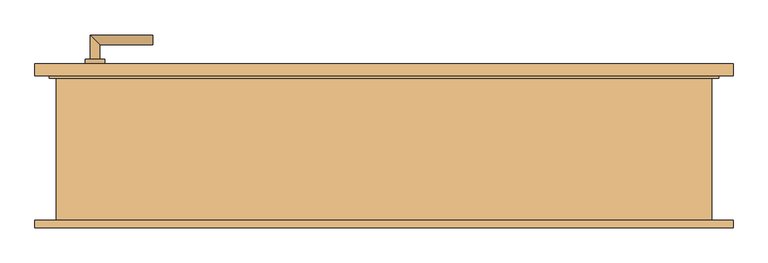
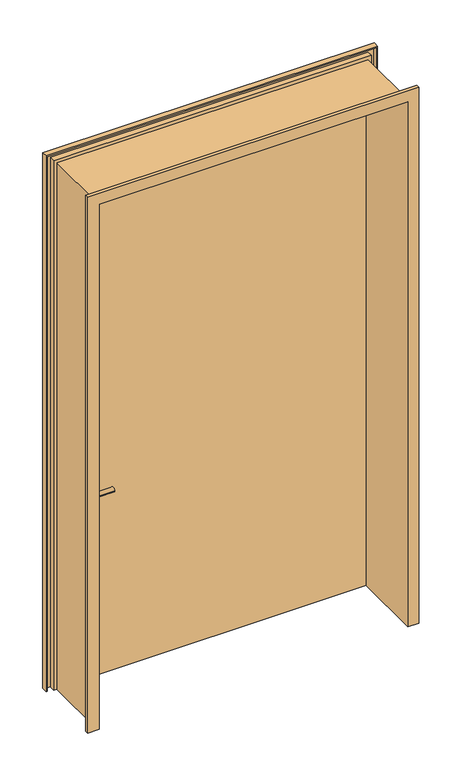
"""IFC4 building model written with IfcOpenShell, lengths in millimetres: door geometry, Drehflügel 1-flg - Stahlzarge : Holztüre 1,4 x 2,45 2."""

import ifcopenshell
import ifcopenshell.guid

model = None  # the IFC model being written
_history = None  # IfcOwnerHistory: only IFC2X3 demands one
_inside = {}  # id of a spatial element -> (the spatial element, [elements in it])
_under = {}  # id of a project, library or spatial element -> (it, [spatial elements below it])
_declared = {}  # id of a project -> (the project, [libraries it declares])
_typed = {}  # id of a type object -> (the type object, [elements of that type])
_made_of = {}  # id of a material, layer set ... -> (it, [elements and type objects made of it])


def new_model(schema):
    """Start an empty IFC model of exactly this schema.

    Asked for "IFC4X3", IfcOpenShell would pick the latest addendum, in which some entities
    have other attributes; the version numbers below select the first issue.
    IFC2X3 requires an IfcOwnerHistory on every rooted entity: one is made here for all.
    """
    global model, _history
    if schema == "IFC4X3":
        model = ifcopenshell.file(schema_version=(4, 3, 0, 0))
    else:
        model = ifcopenshell.file(schema=schema)
    _inside.clear()
    _under.clear()
    _declared.clear()
    _typed.clear()
    _made_of.clear()
    _history = None
    if model.schema == "IFC2X3":
        org = make("IfcOrganization", Name="unknown")
        user = make(
            "IfcPersonAndOrganization",
            ThePerson=make("IfcPerson", FamilyName="unknown"),
            TheOrganization=org,
        )
        app = make(
            "IfcApplication",
            ApplicationDeveloper=org,
            Version="unknown",
            ApplicationFullName="unknown",
            ApplicationIdentifier="unknown",
        )
        _history = make(
            "IfcOwnerHistory",
            OwningUser=user,
            OwningApplication=app,
            ChangeAction="ADDED",
            CreationDate=0,
        )
    return model


def make(cls, **values):
    """One entity of the class cls with the attributes given. An attribute that is None is left unset."""
    return model.create_entity(
        cls, **{name: value for name, value in values.items() if value is not None}
    )


def rooted(cls, **values):
    """An entity with a GlobalId (a new one), such as an element, a storey or a relation."""
    return make(cls, GlobalId=ifcopenshell.guid.new(), OwnerHistory=_history, **values)


def si_unit(unit_type, name, prefix=None):
    """IfcSIUnit, for example si_unit("LENGTHUNIT", "METRE", prefix="MILLI")."""
    return make("IfcSIUnit", UnitType=unit_type, Prefix=prefix, Name=name)


def assignment(units):
    """IfcUnitAssignment: the units of a project."""
    return None if units is None else make("IfcUnitAssignment", Units=units)


def point(xyz):
    """IfcCartesianPoint."""
    return None if xyz is None else make("IfcCartesianPoint", Coordinates=xyz)


def direction(xyz):
    """IfcDirection."""
    return None if xyz is None else make("IfcDirection", DirectionRatios=xyz)


def frame(location, z_axis=None, x_axis=None):
    """IfcAxis2Placement3D, a coordinate frame: its origin and axes. An axis left out is left unset."""
    return make(
        "IfcAxis2Placement3D",
        Location=point(location),
        Axis=direction(z_axis),
        RefDirection=direction(x_axis),
    )


def frame_2d(location, x_axis=None):
    """IfcAxis2Placement2D, a coordinate frame in the plane: its origin and x axis."""
    return make(
        "IfcAxis2Placement2D", Location=point(location), RefDirection=direction(x_axis)
    )


def origin():
    """The frame at (0, 0, 0) with its axes left unset."""
    return frame((0.0, 0.0, 0.0))


def place(relative_to, where):
    """IfcLocalPlacement: puts the frame where relative to a parent placement (None: the world)."""
    return make(
        "IfcLocalPlacement", PlacementRelTo=relative_to, RelativePlacement=where
    )


def context(
    kind, dimensions, precision=None, world=None, true_north=None, identifier=None
):
    """IfcGeometricRepresentationContext, for example the 3D "Model" context."""
    return make(
        "IfcGeometricRepresentationContext",
        ContextIdentifier=identifier,
        ContextType=kind,
        CoordinateSpaceDimension=dimensions,
        Precision=precision,
        WorldCoordinateSystem=world,
        TrueNorth=true_north,
    )


def project(units=None, contexts=None):
    """IfcProject with its units and contexts."""
    return rooted(
        "IfcProject",
        Name="project",
        RepresentationContexts=contexts,
        UnitsInContext=assignment(units),
    )


def spatial(cls, under=None, at=None, **own):
    """A site, building, storey or space (cls), placed at a placement, below another one or the project."""
    s = rooted(cls, ObjectPlacement=at, **own)
    if under is not None:
        _under.setdefault(under.id(), (under, []))[1].append(s)
    return s


def polyline(points):
    """IfcPolyline through the points."""
    return make("IfcPolyline", Points=[point(p) for p in points])


def circle_curve(where, radius):
    """IfcCircle in the frame where."""
    return make("IfcCircle", Position=where, Radius=radius)


def ellipse_curve(where, semi_axis1, semi_axis2):
    """IfcEllipse in the frame where."""
    return make(
        "IfcEllipse", Position=where, SemiAxis1=semi_axis1, SemiAxis2=semi_axis2
    )


def trimmed(basis, trim1, trim2, sense, master):
    """IfcTrimmedCurve: the piece of a basis curve between two trims."""
    return make(
        "IfcTrimmedCurve",
        BasisCurve=basis,
        Trim1=trim1,
        Trim2=trim2,
        SenseAgreement=sense,
        MasterRepresentation=master,
    )


def segment(curve, same_sense, transition):
    """IfcCompositeCurveSegment."""
    return make(
        "IfcCompositeCurveSegment",
        Transition=transition,
        SameSense=same_sense,
        ParentCurve=curve,
    )


def composite_curve(segments, self_intersect=None):
    """IfcCompositeCurve: segments joined end to end."""
    return make("IfcCompositeCurve", Segments=segments, SelfIntersect=self_intersect)


def outline(outer, holes=None, kind="AREA"):
    """IfcArbitraryClosedProfileDef: a profile drawn as a closed curve; with holes, ...WithVoids."""
    if holes is None:
        return make("IfcArbitraryClosedProfileDef", ProfileType=kind, OuterCurve=outer)
    return make(
        "IfcArbitraryProfileDefWithVoids",
        ProfileType=kind,
        OuterCurve=outer,
        InnerCurves=holes,
    )


def extrude(swept, where, along, depth):
    """IfcExtrudedAreaSolid: the profile swept, set in the frame where, extruded along a direction by depth."""
    return make(
        "IfcExtrudedAreaSolid",
        SweptArea=swept,
        Position=where,
        ExtrudedDirection=direction(along),
        Depth=depth,
    )


def faces_of(points, faces, orient=None, outer=None):
    """IfcFace entities. A face is a list of loops; a loop is a list of indices into points, from 0.

    orient and outer hold one flag for each loop. By default every Orientation is true, the
    first loop of a face is its IfcFaceOuterBound and the others are IfcFaceBound.
    """
    made = []
    for i, loops in enumerate(faces):
        bounds = []
        for j, loop in enumerate(loops):
            is_outer = j == 0 if outer is None else outer[i][j]
            bounds.append(
                make(
                    "IfcFaceOuterBound" if is_outer else "IfcFaceBound",
                    Bound=make("IfcPolyLoop", Polygon=[points[k] for k in loop]),
                    Orientation=True if orient is None else orient[i][j],
                )
            )
        made.append(make("IfcFace", Bounds=bounds))
    return made


def faceted_brep(points, faces, orient=None, outer=None, voids=None):
    """IfcFacetedBrep: a solid bounded by flat faces; with voids (closed shells), ...WithVoids."""
    shared = [point(p) for p in points]
    hull = make("IfcClosedShell", CfsFaces=faces_of(shared, faces, orient, outer))
    if voids is None:
        return make("IfcFacetedBrep", Outer=hull)
    return make(
        "IfcFacetedBrepWithVoids",
        Outer=hull,
        Voids=[
            make(cls, CfsFaces=faces_of(shared, fs, o, b)) for cls, fs, o, b in voids
        ],
    )


def shape(context_of_items, identifier, shape_type, items):
    """IfcShapeRepresentation: the items that make up one representation, for example the "Body"."""
    return make(
        "IfcShapeRepresentation",
        ContextOfItems=context_of_items,
        RepresentationIdentifier=identifier,
        RepresentationType=shape_type,
        Items=items,
    )


def source(mapping_origin, context_of_items, identifier, shape_type, items):
    """IfcRepresentationMap: a shape defined once, which mapped items show again and again."""
    return make(
        "IfcRepresentationMap",
        MappingOrigin=mapping_origin,
        MappedRepresentation=shape(context_of_items, identifier, shape_type, items),
    )


def transform(
    local_origin,
    x_axis=None,
    y_axis=None,
    z_axis=None,
    scale=None,
    scale2=None,
    scale3=None,
    uniform=True,
):
    """IfcCartesianTransformationOperator3D, or its non-uniform kind. x_axis, y_axis, z_axis: its Axis1, 2, 3."""
    if uniform:
        return make(
            "IfcCartesianTransformationOperator3D",
            Axis1=direction(x_axis),
            Axis2=direction(y_axis),
            LocalOrigin=point(local_origin),
            Scale=scale,
            Axis3=direction(z_axis),
        )
    return make(
        "IfcCartesianTransformationOperator3DnonUniform",
        Axis1=direction(x_axis),
        Axis2=direction(y_axis),
        LocalOrigin=point(local_origin),
        Scale=scale,
        Axis3=direction(z_axis),
        Scale2=scale2,
        Scale3=scale3,
    )


def mapped(mapping_source, mapping_target):
    """IfcMappedItem: shows the shape of a source again, moved by a transform."""
    return make(
        "IfcMappedItem", MappingSource=mapping_source, MappingTarget=mapping_target
    )


def made_of(thing, what):
    """Note that an element or type object is made of a material, layer set ...; save() writes the relation."""
    if what is not None:
        _made_of.setdefault(what.id(), (what, []))[1].append(thing)
    return thing


def element(
    cls,
    number,
    at=None,
    inside=None,
    cuts=None,
    type_object=None,
    material=None,
    context=None,
    identifier="Body",
    shape_type=None,
    held_by="IfcProductDefinitionShape",
    body=None,
    shapes=None,
    **own,
):
    """One element of the class cls, such as IfcWall. Its Tag is "e" and its number.

    at: its placement. inside: the storey or other place that contains it. cuts: it is an
    opening in that element (IfcRelVoidsElement). A single representation is given by context,
    identifier, shape_type and body (its items); several are given by shapes. held_by: the class
    of the entity that holds the representations. save() writes the other relations.
    """
    e = rooted(cls, Tag="e%d" % number, ObjectPlacement=at, **own)
    if body is not None:
        shapes = [shape(context, identifier, shape_type, body)]
    if shapes is not None:
        e.Representation = make(held_by, Representations=shapes)
    if inside is not None:
        _inside.setdefault(inside.id(), (inside, []))[1].append(e)
    if cuts is not None:
        rooted(
            "IfcRelVoidsElement", RelatingBuildingElement=cuts, RelatedOpeningElement=e
        )
    if type_object is not None:
        _typed.setdefault(type_object.id(), (type_object, []))[1].append(e)
    return made_of(e, material)


def aggregate(whole, parts):
    """IfcRelAggregates: a whole, such as a stair, and the parts it consists of."""
    return rooted("IfcRelAggregates", RelatingObject=whole, RelatedObjects=parts)


def save(model, path):
    """Write the relations noted so far, then the file.

    IfcRelAggregates (storeys below a building ...), IfcRelContainedInSpatialStructure (elements
    in a storey), IfcRelDefinesByType, IfcRelAssociatesMaterial and IfcRelDeclares: one each for
    every whole, place, type object, material and project.
    """
    for whole, parts in _under.values():
        aggregate(whole, parts)
    for where, things in _inside.values():
        rooted(
            "IfcRelContainedInSpatialStructure",
            RelatedElements=things,
            RelatingStructure=where,
        )
    for kind, things in _typed.values():
        rooted("IfcRelDefinesByType", RelatedObjects=things, RelatingType=kind)
    for what, things in _made_of.values():
        rooted("IfcRelAssociatesMaterial", RelatedObjects=things, RelatingMaterial=what)
    for by, libraries in _declared.values():
        rooted("IfcRelDeclares", RelatingContext=by, RelatedDefinitions=libraries)
    model.write(path)


def plane_surface(at):
    """IfcPlane: the flat surface through the origin of the frame at, square to its z axis."""
    return make("IfcPlane", Position=at)


def cylinder_surface(at, radius):
    """IfcCylindricalSurface: all points at the distance radius from the z axis of the frame at."""
    return make("IfcCylindricalSurface", Position=at, Radius=radius)


def advanced_brep(points, edges, surfaces, faces):
    """IfcAdvancedBrep: a solid bounded by faces that lie on surfaces and meet in shared edges.

    An edge is (start, end): straight between two places in points (the first is 0);
    or (start, end, curve); or (start, end, curve, False) where it runs against its curve.
    A face is (place in surfaces, loops), or (place, loops, False) where it looks against
    its surface's normal. A loop lists edges by number (the first is 1), with a minus sign
    where the edge is run from its end to its start. The first loop is the outer one.
    """
    corners = [point(p) for p in points]
    vertices = [make("IfcVertexPoint", VertexGeometry=c) for c in corners]
    made = []
    for start, end, *more in edges:
        made.append(
            make(
                "IfcEdgeCurve",
                EdgeStart=vertices[start],
                EdgeEnd=vertices[end],
                EdgeGeometry=more[0] if more else make("IfcPolyline", Points=[corners[start], corners[end]]),
                SameSense=more[1] if len(more) > 1 else True,
            )
        )
    hull = []
    for where, loops, *sense in faces:
        bounds = []
        for j, loop in enumerate(loops):
            ring = [make("IfcOrientedEdge", EdgeElement=made[abs(k) - 1], Orientation=k > 0) for k in loop]
            bounds.append(
                make(
                    "IfcFaceOuterBound" if j == 0 else "IfcFaceBound",
                    Bound=make("IfcEdgeLoop", EdgeList=ring),
                    Orientation=True,
                )
            )
        hull.append(make("IfcAdvancedFace", Bounds=bounds, FaceSurface=surfaces[where], SameSense=sense[0] if sense else True))
    return make("IfcAdvancedBrep", Outer=make("IfcClosedShell", CfsFaces=hull))


def door_901329f2(model_context):
    return source(origin(), model_context, "Body", "SolidModel", [
        advanced_brep(
        [(-610.0, 139.4346141, 1000.0), (-590.0, 139.4346141, 1000.0), (-610.0, 69.4346141, 1000.0), (-590.0, 89.4346141, 1000.0), (-480.0, 69.4346141, 1000.0), (-480.0, 89.4346141, 1000.0)],
        [
            (0, 1, circle_curve(frame((-600.0, 139.4346141, 1000.0), z_axis=(0.0, 1.0, 0.0), x_axis=(1.0, 0.0, 0.0)), 10.0)),
            (1, 0, circle_curve(frame((-600.0, 139.4346141, 1000.0), z_axis=(0.0, 1.0, 0.0), x_axis=(1.0, 0.0, 0.0)), 10.0)),
            (0, 2),
            (2, 3, ellipse_curve(frame((-600.0, 79.4346141, 1000.0), z_axis=(-0.7071067811865385, 0.7071067811865565, 0.0), x_axis=(0.7071067811865563, 0.7071067811865386, 0.0)), 14.1421356, 10.0)),
            (3, 1),
            (3, 2, ellipse_curve(frame((-600.0, 79.4346141, 1000.0), z_axis=(-0.7071067811865385, 0.7071067811865565, 0.0), x_axis=(0.7071067811865563, 0.7071067811865386, 0.0)), 14.1421356, 10.0)),
            (4, 5, circle_curve(frame((-480.0, 79.4346141, 1000.0), z_axis=(1.0, 0.0, 0.0), x_axis=(0.0, 1.0, 0.0)), 10.0)),
            (5, 4, circle_curve(frame((-480.0, 79.4346141, 1000.0), z_axis=(1.0, 0.0, 0.0), x_axis=(0.0, 1.0, 0.0)), 10.0)),
            (2, 4),
            (5, 3),
        ],
        [
            plane_surface(frame((-600.0, 139.4346141, -287.7526403), z_axis=(0.0, 1.0, 0.0), x_axis=(0.0, 0.0, 1.0))),
            cylinder_surface(frame((-600.0, 139.4346141, 1000.0), z_axis=(0.0, 1.0, 0.0), x_axis=(1.0, 0.0, 0.0)), 10.0),
            plane_surface(frame((-480.0, 79.4346141, -287.7526403), z_axis=(1.0, 0.0, 0.0), x_axis=(0.0, 0.0, 1.0))),
            cylinder_surface(frame((-600.0, 79.4346141, 1000.0), z_axis=(-1.0, 0.0, 0.0), x_axis=(0.0, 1.0, 0.0)), 10.0),
        ],
        [
            (0, [[1, 2]]),
            (1, [[-1, 3, 4, 5]]),
            (1, [[-2, -5, 6, -3]]),
            (2, [[7, 8]]),
            (3, [[-4, 9, -8, 10]]),
            (3, [[-6, -10, -7, -9]]),
        ],
    ),
        advanced_brep(
        [(-590.0, 199.4346141, 1000.0), (-610.0, 199.4346141, 1000.0), (-590.0, 229.4346141, 1000.0), (-610.0, 249.4346141, 1000.0), (-480.0, 229.4346141, 1000.0), (-480.0, 249.4346141, 1000.0)],
        [
            (0, 1, circle_curve(frame((-600.0, 199.4346141, 1000.0), z_axis=(0.0, -1.0, 0.0), x_axis=(-1.0, 0.0, 0.0)), 10.0)),
            (1, 0, circle_curve(frame((-600.0, 199.4346141, 1000.0), z_axis=(0.0, -1.0, 0.0), x_axis=(-1.0, 0.0, 0.0)), 10.0)),
            (0, 2),
            (2, 3, ellipse_curve(frame((-600.0, 239.4346141, 1000.0), z_axis=(-0.7071067811865475, -0.7071067811865475, 0.0), x_axis=(0.7071067811865474, -0.7071067811865476, 0.0)), 14.1421356, 10.0)),
            (3, 1),
            (3, 2, ellipse_curve(frame((-600.0, 239.4346141, 1000.0), z_axis=(-0.7071067811865475, -0.7071067811865475, 0.0), x_axis=(0.7071067811865474, -0.7071067811865476, 0.0)), 14.1421356, 10.0)),
            (4, 5, circle_curve(frame((-480.0, 239.4346141, 1000.0), z_axis=(1.0, 0.0, 0.0), x_axis=(0.0, 1.0, 0.0)), 10.0)),
            (5, 4, circle_curve(frame((-480.0, 239.4346141, 1000.0), z_axis=(1.0, 0.0, 0.0), x_axis=(0.0, 1.0, 0.0)), 10.0)),
            (2, 4),
            (5, 3),
        ],
        [
            plane_surface(frame((-600.0, 199.4346141, -287.7526403), z_axis=(0.0, -1.0, 0.0), x_axis=(0.0, 0.0, 1.0))),
            cylinder_surface(frame((-600.0, 199.4346141, 1000.0), z_axis=(0.0, -1.0, 0.0), x_axis=(-1.0, 0.0, 0.0)), 10.0),
            plane_surface(frame((-480.0, 239.4346141, -287.7526403), z_axis=(1.0, 0.0, 0.0), x_axis=(0.0, 0.0, 1.0))),
            cylinder_surface(frame((-600.0, 239.4346141, 1000.0), z_axis=(-1.0, 0.0, 0.0), x_axis=(0.0, 1.0, 0.0)), 10.0),
        ],
        [
            (0, [[1, 2]]),
            (1, [[-1, 3, 4, 5]]),
            (1, [[-2, -5, 6, -3]]),
            (2, [[7, 8]]),
            (3, [[-4, 9, -8, 10]]),
            (3, [[-6, -10, -7, -9]]),
        ],
    ),
        extrude(outline(composite_curve([segment(trimmed(circle_curve(frame_2d((1000.0, -600.0)), 20.0), [point((1000.0, -620.0))], [point((1000.0, -580.0))], False, "CARTESIAN"), True, "CONTINUOUS"), segment(trimmed(circle_curve(frame_2d((1000.0, -600.0)), 20.0), [point((1000.0, -580.0))], [point((1000.0, -620.0))], False, "CARTESIAN"), True, "CONTINUOUS")], self_intersect=False)), frame((0.0, 129.4346141, 0.0), z_axis=(0.0, 1.0, 0.0), x_axis=(0.0, 0.0, 1.0)), (0.0, 0.0, 1.0), 10.0),
        extrude(outline(composite_curve([segment(trimmed(circle_curve(frame_2d((1000.0, -600.0)), 20.0), [point((1000.0, -620.0))], [point((1000.0, -580.0))], False, "CARTESIAN"), True, "CONTINUOUS"), segment(trimmed(circle_curve(frame_2d((1000.0, -600.0)), 20.0), [point((1000.0, -580.0))], [point((1000.0, -620.0))], False, "CARTESIAN"), True, "CONTINUOUS")], self_intersect=False)), frame((0.0, 189.4346141, 0.0), z_axis=(0.0, 1.0, 0.0), x_axis=(0.0, 0.0, 1.0)), (0.0, 0.0, 1.0), 10.0),
        extrude(outline(polyline([(690.0, 164.4346141), (-690.0, 164.4346141), (-690.0, 189.4346141), (690.0, 189.4346141), (690.0, 164.4346141)])), frame((0.0, 0.0, 100.0), z_axis=(0.0, 0.0, 1.0), x_axis=(1.0, 0.0, 0.0)), (0.0, 0.0, 1.0), 2440.0),
        faceted_brep([(724.4603207, -150.5653859, 100.0), (675.0, -150.5653859, 100.0), (675.0, 164.4346141, 100.0), (690.0, 164.4346141, 100.0), (690.0, 189.4346141, 100.0), (724.4603207, 189.4346141, 100.0), (724.4603207, 164.4346141, 100.0), (719.4603207, 164.4346141, 100.0), (719.4603207, 184.4346141, 100.0), (695.0, 184.4346141, 100.0), (695.0, 159.4346141, 100.0), (680.0, 159.4346141, 100.0), (680.0, -145.5653859, 100.0), (719.4603207, -145.5653859, 100.0), (719.4603207, -135.5653859, 100.0), (724.4603207, -135.5653859, 100.0), (724.4603207, -150.5653859, 2574.4603207), (-724.4603207, -150.5653859, 2574.4603207), (-724.4603207, -150.5653859, 100.0), (-675.0, -150.5653859, 100.0), (-675.0, -150.5653859, 2525.0), (675.0, -150.5653859, 2525.0), (675.0, 164.4346141, 2525.0), (-675.0, 164.4346141, 2525.0), (-675.0, 164.4346141, 100.0), (-690.0, 164.4346141, 100.0), (-690.0, 164.4346141, 2540.0), (690.0, 164.4346141, 2540.0), (690.0, 189.4346141, 2540.0), (-690.0, 189.4346141, 2540.0), (-690.0, 189.4346141, 100.0), (-724.4603207, 189.4346141, 100.0), (-724.4603207, 189.4346141, 2574.4603207), (724.4603207, 189.4346141, 2574.4603207), (724.4603207, 164.4346141, 2574.4603207), (-724.4603207, 164.4346141, 2574.4603207), (-724.4603207, 164.4346141, 100.0), (-719.4603207, 164.4346141, 100.0), (-719.4603207, 164.4346141, 2569.4603207), (719.4603207, 164.4346141, 2569.4603207), (719.4603207, 184.4346141, 2569.4603207), (-719.4603207, 184.4346141, 2569.4603207), (-719.4603207, 184.4346141, 100.0), (-695.0, 184.4346141, 100.0), (-695.0, 184.4346141, 2545.0), (695.0, 184.4346141, 2545.0), (695.0, 159.4346141, 2545.0), (-695.0, 159.4346141, 2545.0), (-695.0, 159.4346141, 100.0), (-680.0, 159.4346141, 100.0), (-680.0, 159.4346141, 2530.0), (680.0, 159.4346141, 2530.0), (680.0, -145.5653859, 2530.0), (-680.0, -145.5653859, 2530.0), (-680.0, -145.5653859, 100.0), (-719.4603207, -145.5653859, 100.0), (-719.4603207, -145.5653859, 2569.4603207), (719.4603207, -145.5653859, 2569.4603207), (719.4603207, -135.5653859, 2569.4603207), (-719.4603207, -135.5653859, 2569.4603207), (-719.4603207, -135.5653859, 100.0), (-724.4603207, -135.5653859, 100.0), (-724.4603207, -135.5653859, 2574.4603207), (724.4603207, -135.5653859, 2574.4603207)], [[[0, 1, 2, 3, 4, 5, 6, 7, 8, 9, 10, 11, 12, 13, 14, 15]], [[1, 0, 16, 17, 18, 19, 20, 21]], [[2, 1, 21, 22]], [[3, 2, 22, 23, 24, 25, 26, 27]], [[4, 3, 27, 28]], [[5, 4, 28, 29, 30, 31, 32, 33]], [[6, 5, 33, 34]], [[7, 6, 34, 35, 36, 37, 38, 39]], [[8, 7, 39, 40]], [[9, 8, 40, 41, 42, 43, 44, 45]], [[10, 9, 45, 46]], [[11, 10, 46, 47, 48, 49, 50, 51]], [[12, 11, 51, 52]], [[13, 12, 52, 53, 54, 55, 56, 57]], [[14, 13, 57, 58]], [[15, 14, 58, 59, 60, 61, 62, 63]], [[0, 15, 63, 16]], [[17, 62, 61, 18]], [[18, 61, 60, 55, 54, 49, 48, 43, 42, 37, 36, 31, 30, 25, 24, 19]], [[23, 20, 19, 24]], [[29, 26, 25, 30]], [[35, 32, 31, 36]], [[41, 38, 37, 42]], [[47, 44, 43, 48]], [[53, 50, 49, 54]], [[59, 56, 55, 60]], [[22, 21, 20, 23]], [[28, 27, 26, 29]], [[34, 33, 32, 35]], [[40, 39, 38, 41]], [[46, 45, 44, 47]], [[52, 51, 50, 53]], [[58, 57, 56, 59]], [[16, 63, 62, 17]]]),
    ])


if __name__ == "__main__":
    model = new_model("IFC4")
    model_context = context("Model", 3, world=origin())
    ifc_project = project(units=[si_unit("LENGTHUNIT", "METRE", prefix="MILLI")], contexts=[model_context])
    site = spatial("IfcSite", under=ifc_project)
    building = spatial("IfcBuilding", under=site)
    placement = place(None, origin())
    door_shape = door_901329f2(model_context)
    element("IfcDoor", 1, ObjectType="Drehflügel 1-flg - Stahlzarge : Holztüre 1,4 x 2,45 2", at=placement, inside=building, context=model_context, shape_type="MappedRepresentation", body=[
        mapped(door_shape, transform((0.0, 0.0, 0.0), x_axis=(1.0, 0.0, 0.0), y_axis=(0.0, 1.0, 0.0), z_axis=(0.0, 0.0, 1.0))),
    ])
    save(model, "model.ifc")

# Revit data of these elements
# Type "Drehflügel 1-flg - Stahlzarge : Holztüre 1,4 x 2,45 2"
#   Type Mark = "24"
#   Operation = "SingleSwingRight"
#   Keynote = "16.03"
#   Analytic Construction = "Metall"
#   Thermal Resistance (R) = 0.270117 (m²·K)/W
#   Heat Transfer Coefficient (U) = 3.7021 W/(m²·K)
#   Rough Width = 1.400 m
#   Rough Height [instance default] = 2.550 m
#   Höhe Türgriff [instance default] = 0.900 m
#   Height = 2.450 m
#   Fußbodenaufbau [instance default] = 0.100 m
#   Width = 1.400 m
#   Sichtbarkeit Sturzlinien [instance default] = yes
#   Türgriff auswählen [instance default] = element 221079
#   Türgriff [instance default] = none
#   Türflügel [instance default] = none
#   Rahmen/Pfosten [instance default] = Metall - Lackiert - Grau
#   Visual Light Transmittance = 0
#   Solar Heat Gain Coefficient = 0
#   Function = (empty or 0)
#   Wall Closure = (empty or 0)
# Element 1 (IfcDoor, "Drehflügel 1-flg - Stahlzarge : Holztüre 1,4 x 2,45 2")
#   Rahmen/Pfosten = Holz - Eiche
#   Materials on its faces: "Holz - Eiche", "Metall - Chrom", "Holz - Birke"
# Materials
#   "Metall - Lackiert - Grau": class "Farbe 1", colour RGB 98 98 98, transparency 0, Cost = 0
#   "Holz - Eiche": class "Holz", colour RGB 151 89 53, transparency 0, Cost = 0
#   "Metall - Chrom": class "Metall", colour RGB 247 247 247, transparency 0, Cost = 0
#   "Holz - Birke": class "Holz", colour RGB 213 164 103, transparency 0, Cost = 0
